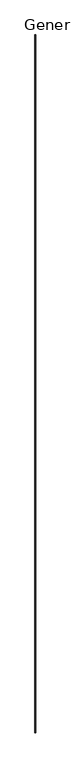
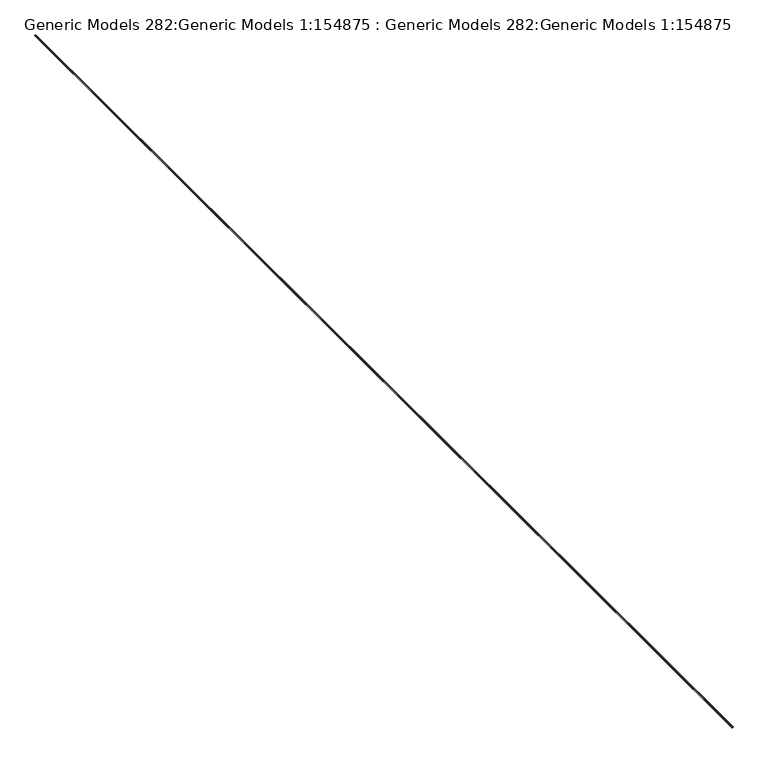
"""IFC4 building model written with IfcOpenShell, lengths in millimetres: proxy geometry, Generic Models 282:Generic Models 1:154875 : Generic Models 282:Generic Models 1:154875."""

from ifc_helpers import new_model, si_unit, point, frame, frame_2d, origin, place, context, project, spatial, polyline, circle_curve, trimmed, segment, composite_curve, outline, extrude, source, transform, mapped, element, save


def generic_models_282_generic_models_1_154875_generic_models_4e7edec8(model_context):
    return source(origin(), model_context, "Body", "SweptSolid", [
        extrude(outline(composite_curve([segment(trimmed(circle_curve(frame_2d((5831.6175253, 1476.3261519)), 6.4650413), [point((5836.3800253, 1480.6982627))], [point((5826.8550253, 1480.6982627))], True, "CARTESIAN"), True, "CONTINUOUS"), segment(polyline([(5826.8550253, 1480.6982627), (5826.8550253, 1485.4607627)]), True, "CONTINUOUS"), segment(trimmed(circle_curve(frame_2d((5831.6175253, 1481.0886519)), 6.4650413), [point((5826.8550253, 1485.4607627))], [point((5828.7610132, 1486.8884016))], False, "CARTESIAN"), True, "CONTINUOUS"), segment(polyline([(5828.7610132, 1486.8884016), (5828.0067788, 1487.9463145), (5827.4222903, 1489.2232154), (5827.0350254, 1490.6590755), (5826.8631898, 1492.1863931), (5826.9148617, 1493.7333671), (5827.187612, 1495.2272722), (5827.6686184, 1496.5978779), (5828.3352681, 1497.7807503), (5829.156221, 1498.7202809), (5830.092883, 1499.3723012), (5831.1012205, 1499.7061589), (5832.1338302, 1499.7061589), (5833.1421676, 1499.3723012), (5834.0788297, 1498.7202809), (5834.8997826, 1497.7807503), (5835.5664322, 1496.5978779), (5836.0474386, 1495.2272722), (5836.320189, 1493.7333671), (5836.3718609, 1492.1863931), (5836.2000253, 1490.6590755), (5835.8127603, 1489.2232154), (5835.2282719, 1487.9463145), (5834.4740375, 1486.8884016)]), True, "CONTINUOUS"), segment(trimmed(circle_curve(frame_2d((5831.6175253, 1481.0886519)), 6.4650413), [point((5834.4740375, 1486.8884016))], [point((5836.3800253, 1485.4607627))], False, "CARTESIAN"), True, "CONTINUOUS"), segment(polyline([(5836.3800253, 1485.4607627), (5836.3800253, 1480.6982627)]), True, "CONTINUOUS")], self_intersect=False)), frame((0.0, -7711.8185138, 0.0), z_axis=(0.0, 1.0, 0.0), x_axis=(0.0, 0.0, 1.0)), (0.0, 0.0, 1.0), 19050.0),
    ])


if __name__ == "__main__":
    model = new_model("IFC4")
    model_context = context("Model", 3, world=origin())
    ifc_project = project(units=[si_unit("LENGTHUNIT", "METRE", prefix="MILLI")], contexts=[model_context])
    site = spatial("IfcSite", under=ifc_project)
    building = spatial("IfcBuilding", under=site)
    placement = place(None, origin())
    generic_models_282_generic_models_1_154875_generic_models_shape = generic_models_282_generic_models_1_154875_generic_models_4e7edec8(model_context)
    element("IfcBuildingElementProxy", 1, Name="Generic Models 282:Generic Models 1:154875 : Generic Models 282:Generic Models 1:154875", ObjectType="Generic Models 282:Generic Models 1:154875 : Generic Models 282:Generic Models 1:154875", at=placement, inside=building, context=model_context, shape_type="MappedRepresentation", body=[
        mapped(generic_models_282_generic_models_1_154875_generic_models_shape, transform((0.0, 0.0, 0.0), x_axis=(1.0, 0.0, 0.0), y_axis=(0.0, 1.0, 0.0), z_axis=(0.0, 0.0, 1.0))),
    ])
    save(model, "model.ifc")

# Revit data of these elements
# Type "Generic Models 282:Generic Models 1:154875 : Generic Models 282:Generic Models 1:154875"
#   NameOverride = "Generic Models 282:Generic Models 1:154875"
#   ObjectTypeOverride = "Generic Models 282:Generic Models 1"
#   Reference = "Generic Models 1"
#   Category = "Generic Models"
#   Tag = "154875"
# Element 1 (IfcBuildingElementProxy, "Generic Models 282:Generic Models 1:154875 : Generic Models 282:Generic Models 1:154875")
#   Materials on its faces: "_SEALANT AND BACKROD, IF NECESSARY 12051"
# Materials
#   "_SEALANT AND BACKROD, IF NECESSARY 12051": class "Unassigned", colour RGB 190 220 196, transparency 0
